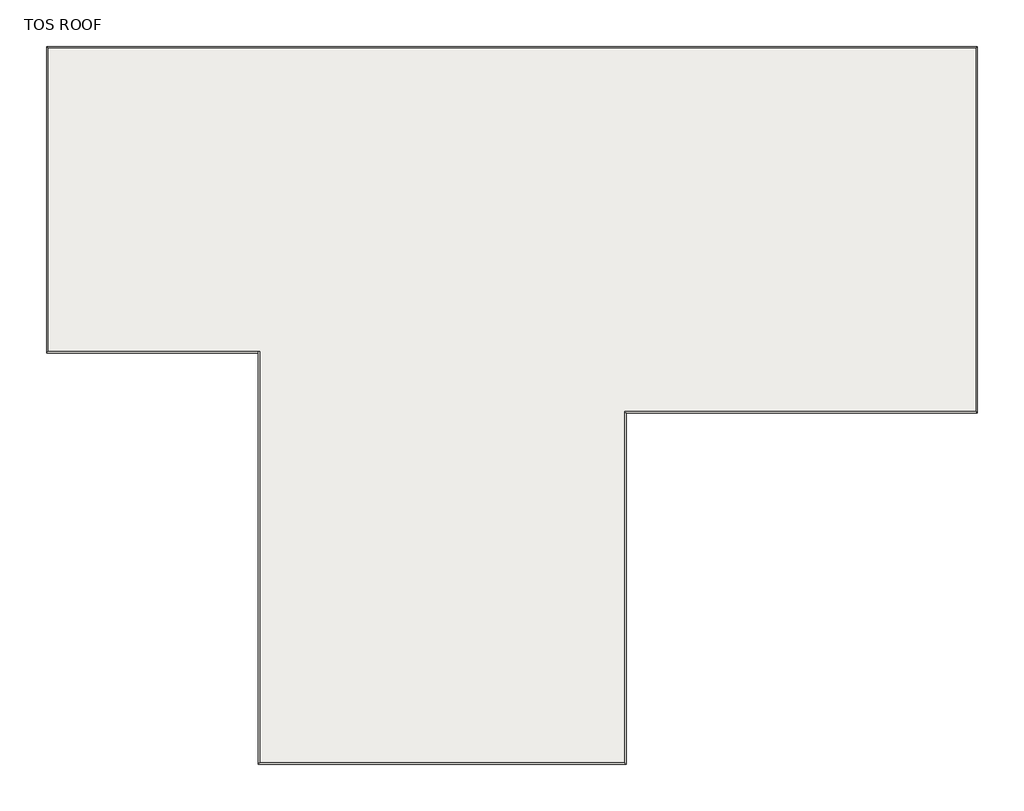
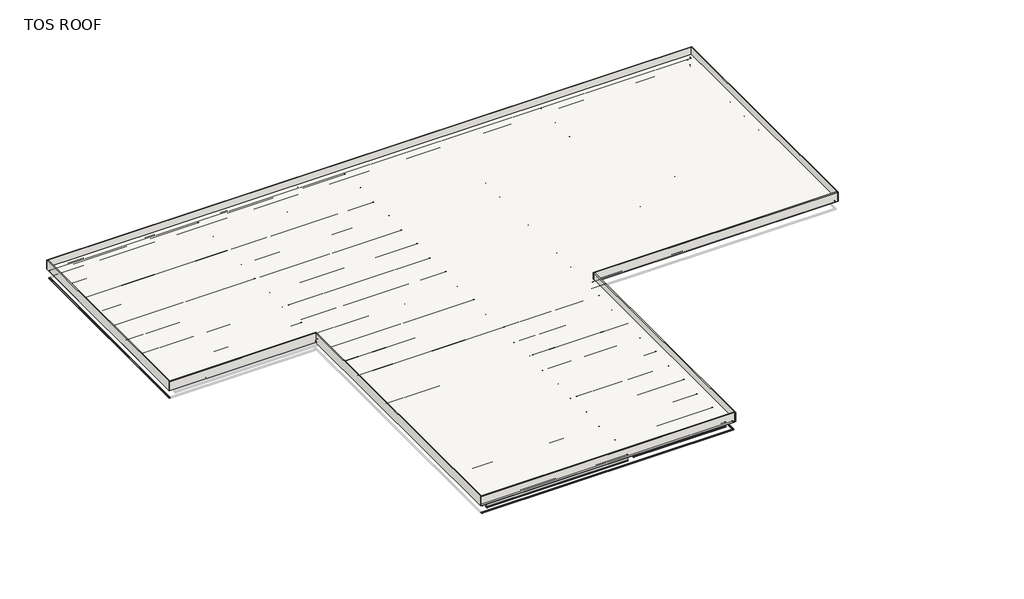
# One storey, part 1 of 3: 41 beams, 8 walls, 1 roof, 1 slab.
"""IFC4 building model written with IfcOpenShell, lengths in millimetres."""

import ifcopenshell
import ifcopenshell.guid

model = None  # the IFC model being written
_history = None  # IfcOwnerHistory: only IFC2X3 demands one
_inside = {}  # id of a spatial element -> (the spatial element, [elements in it])
_under = {}  # id of a project, library or spatial element -> (it, [spatial elements below it])
_declared = {}  # id of a project -> (the project, [libraries it declares])
_typed = {}  # id of a type object -> (the type object, [elements of that type])
_made_of = {}  # id of a material, layer set ... -> (it, [elements and type objects made of it])


def new_model(schema):
    """Start an empty IFC model of exactly this schema.

    Asked for "IFC4X3", IfcOpenShell would pick the latest addendum, in which some entities
    have other attributes; the version numbers below select the first issue.
    IFC2X3 requires an IfcOwnerHistory on every rooted entity: one is made here for all.
    """
    global model, _history
    if schema == "IFC4X3":
        model = ifcopenshell.file(schema_version=(4, 3, 0, 0))
    else:
        model = ifcopenshell.file(schema=schema)
    _inside.clear()
    _under.clear()
    _declared.clear()
    _typed.clear()
    _made_of.clear()
    _history = None
    if model.schema == "IFC2X3":
        org = make("IfcOrganization", Name="unknown")
        user = make(
            "IfcPersonAndOrganization",
            ThePerson=make("IfcPerson", FamilyName="unknown"),
            TheOrganization=org,
        )
        app = make(
            "IfcApplication",
            ApplicationDeveloper=org,
            Version="unknown",
            ApplicationFullName="unknown",
            ApplicationIdentifier="unknown",
        )
        _history = make(
            "IfcOwnerHistory",
            OwningUser=user,
            OwningApplication=app,
            ChangeAction="ADDED",
            CreationDate=0,
        )
    return model


def make(cls, **values):
    """One entity of the class cls with the attributes given. An attribute that is None is left unset."""
    return model.create_entity(
        cls, **{name: value for name, value in values.items() if value is not None}
    )


def rooted(cls, **values):
    """An entity with a GlobalId (a new one), such as an element, a storey or a relation."""
    return make(cls, GlobalId=ifcopenshell.guid.new(), OwnerHistory=_history, **values)


def si_unit(unit_type, name, prefix=None):
    """IfcSIUnit, for example si_unit("LENGTHUNIT", "METRE", prefix="MILLI")."""
    return make("IfcSIUnit", UnitType=unit_type, Prefix=prefix, Name=name)


def assignment(units):
    """IfcUnitAssignment: the units of a project."""
    return None if units is None else make("IfcUnitAssignment", Units=units)


def point(xyz):
    """IfcCartesianPoint."""
    return None if xyz is None else make("IfcCartesianPoint", Coordinates=xyz)


def direction(xyz):
    """IfcDirection."""
    return None if xyz is None else make("IfcDirection", DirectionRatios=xyz)


def frame(location, z_axis=None, x_axis=None):
    """IfcAxis2Placement3D, a coordinate frame: its origin and axes. An axis left out is left unset."""
    return make(
        "IfcAxis2Placement3D",
        Location=point(location),
        Axis=direction(z_axis),
        RefDirection=direction(x_axis),
    )


def frame_2d(location, x_axis=None):
    """IfcAxis2Placement2D, a coordinate frame in the plane: its origin and x axis."""
    return make(
        "IfcAxis2Placement2D", Location=point(location), RefDirection=direction(x_axis)
    )


def origin():
    """The frame at (0, 0, 0) with its axes left unset."""
    return frame((0.0, 0.0, 0.0))


def place(relative_to, where):
    """IfcLocalPlacement: puts the frame where relative to a parent placement (None: the world)."""
    return make(
        "IfcLocalPlacement", PlacementRelTo=relative_to, RelativePlacement=where
    )


def context(
    kind, dimensions, precision=None, world=None, true_north=None, identifier=None
):
    """IfcGeometricRepresentationContext, for example the 3D "Model" context."""
    return make(
        "IfcGeometricRepresentationContext",
        ContextIdentifier=identifier,
        ContextType=kind,
        CoordinateSpaceDimension=dimensions,
        Precision=precision,
        WorldCoordinateSystem=world,
        TrueNorth=true_north,
    )


def project(units=None, contexts=None):
    """IfcProject with its units and contexts."""
    return rooted(
        "IfcProject",
        Name="project",
        RepresentationContexts=contexts,
        UnitsInContext=assignment(units),
    )


def spatial(cls, under=None, at=None, **own):
    """A site, building, storey or space (cls), placed at a placement, below another one or the project."""
    s = rooted(cls, ObjectPlacement=at, **own)
    if under is not None:
        _under.setdefault(under.id(), (under, []))[1].append(s)
    return s


def polyline(points):
    """IfcPolyline through the points."""
    return make("IfcPolyline", Points=[point(p) for p in points])


def circle_curve(where, radius):
    """IfcCircle in the frame where."""
    return make("IfcCircle", Position=where, Radius=radius)


def trimmed(basis, trim1, trim2, sense, master):
    """IfcTrimmedCurve: the piece of a basis curve between two trims."""
    return make(
        "IfcTrimmedCurve",
        BasisCurve=basis,
        Trim1=trim1,
        Trim2=trim2,
        SenseAgreement=sense,
        MasterRepresentation=master,
    )


def segment(curve, same_sense, transition):
    """IfcCompositeCurveSegment."""
    return make(
        "IfcCompositeCurveSegment",
        Transition=transition,
        SameSense=same_sense,
        ParentCurve=curve,
    )


def composite_curve(segments, self_intersect=None):
    """IfcCompositeCurve: segments joined end to end."""
    return make("IfcCompositeCurve", Segments=segments, SelfIntersect=self_intersect)


def outline(outer, holes=None, kind="AREA"):
    """IfcArbitraryClosedProfileDef: a profile drawn as a closed curve; with holes, ...WithVoids."""
    if holes is None:
        return make("IfcArbitraryClosedProfileDef", ProfileType=kind, OuterCurve=outer)
    return make(
        "IfcArbitraryProfileDefWithVoids",
        ProfileType=kind,
        OuterCurve=outer,
        InnerCurves=holes,
    )


def extrude(swept, where, along, depth):
    """IfcExtrudedAreaSolid: the profile swept, set in the frame where, extruded along a direction by depth."""
    return make(
        "IfcExtrudedAreaSolid",
        SweptArea=swept,
        Position=where,
        ExtrudedDirection=direction(along),
        Depth=depth,
    )


def faces_of(points, faces, orient=None, outer=None):
    """IfcFace entities. A face is a list of loops; a loop is a list of indices into points, from 0.

    orient and outer hold one flag for each loop. By default every Orientation is true, the
    first loop of a face is its IfcFaceOuterBound and the others are IfcFaceBound.
    """
    made = []
    for i, loops in enumerate(faces):
        bounds = []
        for j, loop in enumerate(loops):
            is_outer = j == 0 if outer is None else outer[i][j]
            bounds.append(
                make(
                    "IfcFaceOuterBound" if is_outer else "IfcFaceBound",
                    Bound=make("IfcPolyLoop", Polygon=[points[k] for k in loop]),
                    Orientation=True if orient is None else orient[i][j],
                )
            )
        made.append(make("IfcFace", Bounds=bounds))
    return made


def faceted_brep(points, faces, orient=None, outer=None, voids=None):
    """IfcFacetedBrep: a solid bounded by flat faces; with voids (closed shells), ...WithVoids."""
    shared = [point(p) for p in points]
    hull = make("IfcClosedShell", CfsFaces=faces_of(shared, faces, orient, outer))
    if voids is None:
        return make("IfcFacetedBrep", Outer=hull)
    return make(
        "IfcFacetedBrepWithVoids",
        Outer=hull,
        Voids=[
            make(cls, CfsFaces=faces_of(shared, fs, o, b)) for cls, fs, o, b in voids
        ],
    )


def shape(context_of_items, identifier, shape_type, items):
    """IfcShapeRepresentation: the items that make up one representation, for example the "Body"."""
    return make(
        "IfcShapeRepresentation",
        ContextOfItems=context_of_items,
        RepresentationIdentifier=identifier,
        RepresentationType=shape_type,
        Items=items,
    )


def source(mapping_origin, context_of_items, identifier, shape_type, items):
    """IfcRepresentationMap: a shape defined once, which mapped items show again and again."""
    return make(
        "IfcRepresentationMap",
        MappingOrigin=mapping_origin,
        MappedRepresentation=shape(context_of_items, identifier, shape_type, items),
    )


def transform(
    local_origin,
    x_axis=None,
    y_axis=None,
    z_axis=None,
    scale=None,
    scale2=None,
    scale3=None,
    uniform=True,
):
    """IfcCartesianTransformationOperator3D, or its non-uniform kind. x_axis, y_axis, z_axis: its Axis1, 2, 3."""
    if uniform:
        return make(
            "IfcCartesianTransformationOperator3D",
            Axis1=direction(x_axis),
            Axis2=direction(y_axis),
            LocalOrigin=point(local_origin),
            Scale=scale,
            Axis3=direction(z_axis),
        )
    return make(
        "IfcCartesianTransformationOperator3DnonUniform",
        Axis1=direction(x_axis),
        Axis2=direction(y_axis),
        LocalOrigin=point(local_origin),
        Scale=scale,
        Axis3=direction(z_axis),
        Scale2=scale2,
        Scale3=scale3,
    )


def mapped(mapping_source, mapping_target):
    """IfcMappedItem: shows the shape of a source again, moved by a transform."""
    return make(
        "IfcMappedItem", MappingSource=mapping_source, MappingTarget=mapping_target
    )


def made_of(thing, what):
    """Note that an element or type object is made of a material, layer set ...; save() writes the relation."""
    if what is not None:
        _made_of.setdefault(what.id(), (what, []))[1].append(thing)
    return thing


def element(
    cls,
    number,
    at=None,
    inside=None,
    cuts=None,
    type_object=None,
    material=None,
    context=None,
    identifier="Body",
    shape_type=None,
    held_by="IfcProductDefinitionShape",
    body=None,
    shapes=None,
    **own,
):
    """One element of the class cls, such as IfcWall. Its Tag is "e" and its number.

    at: its placement. inside: the storey or other place that contains it. cuts: it is an
    opening in that element (IfcRelVoidsElement). A single representation is given by context,
    identifier, shape_type and body (its items); several are given by shapes. held_by: the class
    of the entity that holds the representations. save() writes the other relations.
    """
    e = rooted(cls, Tag="e%d" % number, ObjectPlacement=at, **own)
    if body is not None:
        shapes = [shape(context, identifier, shape_type, body)]
    if shapes is not None:
        e.Representation = make(held_by, Representations=shapes)
    if inside is not None:
        _inside.setdefault(inside.id(), (inside, []))[1].append(e)
    if cuts is not None:
        rooted(
            "IfcRelVoidsElement", RelatingBuildingElement=cuts, RelatedOpeningElement=e
        )
    if type_object is not None:
        _typed.setdefault(type_object.id(), (type_object, []))[1].append(e)
    return made_of(e, material)


def aggregate(whole, parts):
    """IfcRelAggregates: a whole, such as a stair, and the parts it consists of."""
    return rooted("IfcRelAggregates", RelatingObject=whole, RelatedObjects=parts)


def save(model, path):
    """Write the relations noted so far, then the file.

    IfcRelAggregates (storeys below a building ...), IfcRelContainedInSpatialStructure (elements
    in a storey), IfcRelDefinesByType, IfcRelAssociatesMaterial and IfcRelDeclares: one each for
    every whole, place, type object, material and project.
    """
    for whole, parts in _under.values():
        aggregate(whole, parts)
    for where, things in _inside.values():
        rooted(
            "IfcRelContainedInSpatialStructure",
            RelatedElements=things,
            RelatingStructure=where,
        )
    for kind, things in _typed.values():
        rooted("IfcRelDefinesByType", RelatedObjects=things, RelatingType=kind)
    for what, things in _made_of.values():
        rooted("IfcRelAssociatesMaterial", RelatedObjects=things, RelatingMaterial=what)
    for by, libraries in _declared.values():
        rooted("IfcRelDeclares", RelatingContext=by, RelatedDefinitions=libraries)
    model.write(path)


def beam_c270cd18(model_context):
    return source(origin(), model_context, "Body", "SweptSolid", [
        extrude(outline(composite_curve([segment(polyline([(75.0, -141.0), (75.0, -150.0), (-75.0, -150.0), (-75.0, -141.0), (-16.25, -141.0)]), True, "CONTINUOUS"), segment(trimmed(circle_curve(frame_2d((-16.25, -128.0)), 13.0), [point((-16.25, -141.0))], [point((-3.25, -128.0))], True, "CARTESIAN"), True, "CONTINUOUS"), segment(polyline([(-3.25, -128.0), (-3.25, 128.0)]), True, "CONTINUOUS"), segment(trimmed(circle_curve(frame_2d((-16.25, 128.0)), 13.0), [point((-3.25, 128.0))], [point((-16.25, 141.0))], True, "CARTESIAN"), True, "CONTINUOUS"), segment(polyline([(-16.25, 141.0), (-75.0, 141.0), (-75.0, 150.0), (75.0, 150.0), (75.0, 141.0), (16.25, 141.0)]), True, "CONTINUOUS"), segment(trimmed(circle_curve(frame_2d((16.25, 128.0)), 13.0), [point((16.25, 141.0))], [point((3.25, 128.0))], True, "CARTESIAN"), True, "CONTINUOUS"), segment(polyline([(3.25, 128.0), (3.25, -128.0)]), True, "CONTINUOUS"), segment(trimmed(circle_curve(frame_2d((16.25, -128.0)), 13.0), [point((3.25, -128.0))], [point((16.25, -141.0))], True, "CARTESIAN"), True, "CONTINUOUS"), segment(polyline([(16.25, -141.0), (75.0, -141.0)]), True, "CONTINUOUS")], self_intersect=False)), frame((-2837.3, 0.0, 0.0), z_axis=(1.0, 0.0, 0.0), x_axis=(0.0, 1.0, 0.0)), (0.0, 0.0, 1.0), 5674.6),
    ])


def beam_0d7a42ae(model_context):
    return source(origin(), model_context, "Body", "SweptSolid", [
        extrude(outline(composite_curve([segment(polyline([(100.0, -283.0), (100.0, -300.0), (-100.0, -300.0), (-100.0, -283.0), (-27.5, -283.0)]), True, "CONTINUOUS"), segment(trimmed(circle_curve(frame_2d((-27.5, -261.0)), 22.0), [point((-27.5, -283.0))], [point((-5.5, -261.0))], True, "CARTESIAN"), True, "CONTINUOUS"), segment(polyline([(-5.5, -261.0), (-5.5, 261.0)]), True, "CONTINUOUS"), segment(trimmed(circle_curve(frame_2d((-27.5, 261.0)), 22.0), [point((-5.5, 261.0))], [point((-27.5, 283.0))], True, "CARTESIAN"), True, "CONTINUOUS"), segment(polyline([(-27.5, 283.0), (-100.0, 283.0), (-100.0, 300.0), (100.0, 300.0), (100.0, 283.0), (27.5, 283.0)]), True, "CONTINUOUS"), segment(trimmed(circle_curve(frame_2d((27.5, 261.0)), 22.0), [point((27.5, 283.0))], [point((5.5, 261.0))], True, "CARTESIAN"), True, "CONTINUOUS"), segment(polyline([(5.5, 261.0), (5.5, -261.0)]), True, "CONTINUOUS"), segment(trimmed(circle_curve(frame_2d((27.5, -261.0)), 22.0), [point((5.5, -261.0))], [point((27.5, -283.0))], True, "CARTESIAN"), True, "CONTINUOUS"), segment(polyline([(27.5, -283.0), (100.0, -283.0)]), True, "CONTINUOUS")], self_intersect=False)), frame((-5912.3, 0.0, 0.0), z_axis=(1.0, 0.0, 0.0), x_axis=(0.0, 1.0, 0.0)), (0.0, 0.0, 1.0), 11749.6),
    ])


def beam_9fd407d8(model_context):
    return source(origin(), model_context, "Body", "SweptSolid", [
        extrude(outline(composite_curve([segment(polyline([(150.0, -374.0), (150.0, -400.0), (-150.0, -400.0), (-150.0, -374.0), (-35.0, -374.0)]), True, "CONTINUOUS"), segment(trimmed(circle_curve(frame_2d((-35.0, -346.0)), 28.0), [point((-35.0, -374.0))], [point((-7.0, -346.0))], True, "CARTESIAN"), True, "CONTINUOUS"), segment(polyline([(-7.0, -346.0), (-7.0, 346.0)]), True, "CONTINUOUS"), segment(trimmed(circle_curve(frame_2d((-35.0, 346.0)), 28.0), [point((-7.0, 346.0))], [point((-35.0, 374.0))], True, "CARTESIAN"), True, "CONTINUOUS"), segment(polyline([(-35.0, 374.0), (-150.0, 374.0), (-150.0, 400.0), (150.0, 400.0), (150.0, 374.0), (35.0, 374.0)]), True, "CONTINUOUS"), segment(trimmed(circle_curve(frame_2d((35.0, 346.0)), 28.0), [point((35.0, 374.0))], [point((7.0, 346.0))], True, "CARTESIAN"), True, "CONTINUOUS"), segment(polyline([(7.0, 346.0), (7.0, -346.0)]), True, "CONTINUOUS"), segment(trimmed(circle_curve(frame_2d((35.0, -346.0)), 28.0), [point((7.0, -346.0))], [point((35.0, -374.0))], True, "CARTESIAN"), True, "CONTINUOUS"), segment(polyline([(35.0, -374.0), (150.0, -374.0)]), True, "CONTINUOUS")], self_intersect=False)), frame((-8837.3, 0.0, 0.0), z_axis=(1.0, 0.0, 0.0), x_axis=(0.0, 1.0, 0.0)), (0.0, 0.0, 1.0), 17749.6),
    ])


def beam_a13b9fc3(model_context):
    return source(origin(), model_context, "Body", "SweptSolid", [
        extrude(outline(composite_curve([segment(polyline([(150.0, -374.0), (150.0, -400.0), (-150.0, -400.0), (-150.0, -374.0), (-35.0, -374.0)]), True, "CONTINUOUS"), segment(trimmed(circle_curve(frame_2d((-35.0, -346.0)), 28.0), [point((-35.0, -374.0))], [point((-7.0, -346.0))], True, "CARTESIAN"), True, "CONTINUOUS"), segment(polyline([(-7.0, -346.0), (-7.0, 346.0)]), True, "CONTINUOUS"), segment(trimmed(circle_curve(frame_2d((-35.0, 346.0)), 28.0), [point((-7.0, 346.0))], [point((-35.0, 374.0))], True, "CARTESIAN"), True, "CONTINUOUS"), segment(polyline([(-35.0, 374.0), (-150.0, 374.0), (-150.0, 400.0), (150.0, 400.0), (150.0, 374.0), (35.0, 374.0)]), True, "CONTINUOUS"), segment(trimmed(circle_curve(frame_2d((35.0, 346.0)), 28.0), [point((35.0, 374.0))], [point((7.0, 346.0))], True, "CARTESIAN"), True, "CONTINUOUS"), segment(polyline([(7.0, 346.0), (7.0, -346.0)]), True, "CONTINUOUS"), segment(trimmed(circle_curve(frame_2d((35.0, -346.0)), 28.0), [point((7.0, -346.0))], [point((35.0, -374.0))], True, "CARTESIAN"), True, "CONTINUOUS"), segment(polyline([(35.0, -374.0), (150.0, -374.0)]), True, "CONTINUOUS")], self_intersect=False)), frame((-8693.3, 0.0, 0.0), z_axis=(1.0, 0.0, 0.0), x_axis=(0.0, 1.0, 0.0)), (0.0, 0.0, 1.0), 17386.6),
    ])


def beam_fedc1a72(model_context):
    return source(origin(), model_context, "Body", "SweptSolid", [
        extrude(outline(composite_curve([segment(polyline([(100.0, -283.0), (100.0, -300.0), (-100.0, -300.0), (-100.0, -283.0), (-27.5, -283.0)]), True, "CONTINUOUS"), segment(trimmed(circle_curve(frame_2d((-27.5, -261.0)), 22.0), [point((-27.5, -283.0))], [point((-5.5, -261.0))], True, "CARTESIAN"), True, "CONTINUOUS"), segment(polyline([(-5.5, -261.0), (-5.5, 261.0)]), True, "CONTINUOUS"), segment(trimmed(circle_curve(frame_2d((-27.5, 261.0)), 22.0), [point((-5.5, 261.0))], [point((-27.5, 283.0))], True, "CARTESIAN"), True, "CONTINUOUS"), segment(polyline([(-27.5, 283.0), (-100.0, 283.0), (-100.0, 300.0), (100.0, 300.0), (100.0, 283.0), (27.5, 283.0)]), True, "CONTINUOUS"), segment(trimmed(circle_curve(frame_2d((27.5, 261.0)), 22.0), [point((27.5, 283.0))], [point((5.5, 261.0))], True, "CARTESIAN"), True, "CONTINUOUS"), segment(polyline([(5.5, 261.0), (5.5, -261.0)]), True, "CONTINUOUS"), segment(trimmed(circle_curve(frame_2d((27.5, -261.0)), 22.0), [point((5.5, -261.0))], [point((27.5, -283.0))], True, "CARTESIAN"), True, "CONTINUOUS"), segment(polyline([(27.5, -283.0), (100.0, -283.0)]), True, "CONTINUOUS")], self_intersect=False)), frame((-5693.3, 0.0, 0.0), z_axis=(1.0, 0.0, 0.0), x_axis=(0.0, 1.0, 0.0)), (0.0, 0.0, 1.0), 11386.6),
    ])


def steel_framing_lc_f9ca99c4(model_context):
    return source(origin(), model_context, "Body", "SweptSolid", [
        extrude(outline(composite_curve([segment(polyline([(18.6, 67.0), (18.6, -67.0)]), True, "CONTINUOUS"), segment(trimmed(circle_curve(frame_2d((10.6, -67.0)), 8.0), [point((18.6, -67.0))], [point((10.6, -75.0))], False, "CARTESIAN"), True, "CONTINUOUS"), segment(polyline([(10.6, -75.0), (-48.4, -75.0)]), True, "CONTINUOUS"), segment(trimmed(circle_curve(frame_2d((-48.4, -67.0)), 8.0), [point((-48.4, -75.0))], [point((-56.4, -67.0))], False, "CARTESIAN"), True, "CONTINUOUS"), segment(polyline([(-56.4, -67.0), (-56.4, -50.0), (-53.2, -50.0), (-53.2, -67.0)]), True, "CONTINUOUS"), segment(trimmed(circle_curve(frame_2d((-48.4, -67.0)), 4.8), [point((-53.2, -67.0))], [point((-48.4, -71.8))], True, "CARTESIAN"), True, "CONTINUOUS"), segment(polyline([(-48.4, -71.8), (10.6, -71.8)]), True, "CONTINUOUS"), segment(trimmed(circle_curve(frame_2d((10.6, -67.0)), 4.8), [point((10.6, -71.8))], [point((15.4, -67.0))], True, "CARTESIAN"), True, "CONTINUOUS"), segment(polyline([(15.4, -67.0), (15.4, 67.0)]), True, "CONTINUOUS"), segment(trimmed(circle_curve(frame_2d((10.6, 67.0)), 4.8), [point((15.4, 67.0))], [point((10.6, 71.8))], True, "CARTESIAN"), True, "CONTINUOUS"), segment(polyline([(10.6, 71.8), (-48.4, 71.8)]), True, "CONTINUOUS"), segment(trimmed(circle_curve(frame_2d((-48.4, 67.0)), 4.8), [point((-48.4, 71.8))], [point((-53.2, 67.0))], True, "CARTESIAN"), True, "CONTINUOUS"), segment(polyline([(-53.2, 67.0), (-53.2, 50.0), (-56.4, 50.0), (-56.4, 67.0)]), True, "CONTINUOUS"), segment(trimmed(circle_curve(frame_2d((-48.4, 67.0)), 8.0), [point((-56.4, 67.0))], [point((-48.4, 75.0))], False, "CARTESIAN"), True, "CONTINUOUS"), segment(polyline([(-48.4, 75.0), (10.6, 75.0)]), True, "CONTINUOUS"), segment(trimmed(circle_curve(frame_2d((10.6, 67.0)), 8.0), [point((10.6, 75.0))], [point((18.6, 67.0))], False, "CARTESIAN"), True, "CONTINUOUS")], self_intersect=False)), frame((-12797.0, 0.0, 0.0), z_axis=(1.0, 0.0, 0.0), x_axis=(0.0, 1.0, 0.0)), (0.0, 0.0, 1.0), 25581.0),
    ])


def steel_framing_lc_7a68255c(model_context):
    return source(origin(), model_context, "Body", "SweptSolid", [
        extrude(outline(composite_curve([segment(polyline([(18.6, 67.0), (18.6, -67.0)]), True, "CONTINUOUS"), segment(trimmed(circle_curve(frame_2d((10.6, -67.0)), 8.0), [point((18.6, -67.0))], [point((10.6, -75.0))], False, "CARTESIAN"), True, "CONTINUOUS"), segment(polyline([(10.6, -75.0), (-48.4, -75.0)]), True, "CONTINUOUS"), segment(trimmed(circle_curve(frame_2d((-48.4, -67.0)), 8.0), [point((-48.4, -75.0))], [point((-56.4, -67.0))], False, "CARTESIAN"), True, "CONTINUOUS"), segment(polyline([(-56.4, -67.0), (-56.4, -50.0), (-53.2, -50.0), (-53.2, -67.0)]), True, "CONTINUOUS"), segment(trimmed(circle_curve(frame_2d((-48.4, -67.0)), 4.8), [point((-53.2, -67.0))], [point((-48.4, -71.8))], True, "CARTESIAN"), True, "CONTINUOUS"), segment(polyline([(-48.4, -71.8), (10.6, -71.8)]), True, "CONTINUOUS"), segment(trimmed(circle_curve(frame_2d((10.6, -67.0)), 4.8), [point((10.6, -71.8))], [point((15.4, -67.0))], True, "CARTESIAN"), True, "CONTINUOUS"), segment(polyline([(15.4, -67.0), (15.4, 67.0)]), True, "CONTINUOUS"), segment(trimmed(circle_curve(frame_2d((10.6, 67.0)), 4.8), [point((15.4, 67.0))], [point((10.6, 71.8))], True, "CARTESIAN"), True, "CONTINUOUS"), segment(polyline([(10.6, 71.8), (-48.4, 71.8)]), True, "CONTINUOUS"), segment(trimmed(circle_curve(frame_2d((-48.4, 67.0)), 4.8), [point((-48.4, 71.8))], [point((-53.2, 67.0))], True, "CARTESIAN"), True, "CONTINUOUS"), segment(polyline([(-53.2, 67.0), (-53.2, 50.0), (-56.4, 50.0), (-56.4, 67.0)]), True, "CONTINUOUS"), segment(trimmed(circle_curve(frame_2d((-48.4, 67.0)), 8.0), [point((-56.4, 67.0))], [point((-48.4, 75.0))], False, "CARTESIAN"), True, "CONTINUOUS"), segment(polyline([(-48.4, 75.0), (10.6, 75.0)]), True, "CONTINUOUS"), segment(trimmed(circle_curve(frame_2d((10.6, 67.0)), 8.0), [point((10.6, 75.0))], [point((18.6, 67.0))], False, "CARTESIAN"), True, "CONTINUOUS")], self_intersect=False)), frame((-15450.0, 0.0, 0.0), z_axis=(1.0, 0.0, 0.0), x_axis=(0.0, 1.0, 0.0)), (0.0, 0.0, 1.0), 30900.0),
    ])


model = new_model("IFC4")

# Units and contexts
model_context = context("Model", 3, world=origin())
ifc_project = project(units=[si_unit("LENGTHUNIT", "METRE", prefix="MILLI")], contexts=[model_context])

# Site, building, storey
site = spatial("IfcSite", under=ifc_project)
building = spatial("IfcBuilding", under=site)
storey = spatial("IfcBuildingStorey", under=building, Name="TOS ROOF", Elevation=10199.9618634)

# Beams
placement = place(None, origin())
element("IfcBeam", 1, at=placement, inside=storey, context=model_context, shape_type="SweptSolid", body=[
    extrude(outline(composite_curve([segment(polyline([(9908.9618634, 36075.0), (9908.9618634, 36016.25)]), True, "CONTINUOUS"), segment(trimmed(circle_curve(frame_2d((9921.9618634, 36016.25)), 13.0), [point((9908.9618634, 36016.25))], [point((9921.9618634, 36003.25))], True, "CARTESIAN"), True, "CONTINUOUS"), segment(polyline([(9921.9618634, 36003.25), (10177.9618634, 36003.25)]), True, "CONTINUOUS"), segment(trimmed(circle_curve(frame_2d((10177.9618634, 36016.25)), 13.0), [point((10177.9618634, 36003.25))], [point((10190.9618634, 36016.25))], True, "CARTESIAN"), True, "CONTINUOUS"), segment(polyline([(10190.9618634, 36016.25), (10190.9618634, 36075.0), (10199.9618634, 36075.0), (10199.9618634, 35925.0), (10190.9618634, 35925.0), (10190.9618634, 35983.75)]), True, "CONTINUOUS"), segment(trimmed(circle_curve(frame_2d((10177.9618634, 35983.75)), 13.0), [point((10190.9618634, 35983.75))], [point((10177.9618634, 35996.75))], True, "CARTESIAN"), True, "CONTINUOUS"), segment(polyline([(10177.9618634, 35996.75), (9921.9618634, 35996.75)]), True, "CONTINUOUS"), segment(trimmed(circle_curve(frame_2d((9921.9618634, 35983.75)), 13.0), [point((9921.9618634, 35996.75))], [point((9908.9618634, 35983.75))], True, "CARTESIAN"), True, "CONTINUOUS"), segment(polyline([(9908.9618634, 35983.75), (9908.9618634, 35925.0), (9899.9618634, 35925.0), (9899.9618634, 36075.0), (9908.9618634, 36075.0)]), True, "CONTINUOUS")], self_intersect=False)), frame((0.0, -35837.3, 0.0), z_axis=(0.0, 1.0, 0.0), x_axis=(0.0, 0.0, 1.0)), (0.0, 0.0, 1.0), 5674.6),
])
element("IfcBeam", 2, at=placement, inside=storey, context=model_context, shape_type="SweptSolid", body=[
    extrude(outline(composite_curve([segment(polyline([(9908.9618634, 36075.0), (9908.9618634, 36016.25)]), True, "CONTINUOUS"), segment(trimmed(circle_curve(frame_2d((9921.9618634, 36016.25)), 13.0), [point((9908.9618634, 36016.25))], [point((9921.9618634, 36003.25))], True, "CARTESIAN"), True, "CONTINUOUS"), segment(polyline([(9921.9618634, 36003.25), (10177.9618634, 36003.25)]), True, "CONTINUOUS"), segment(trimmed(circle_curve(frame_2d((10177.9618634, 36016.25)), 13.0), [point((10177.9618634, 36003.25))], [point((10190.9618634, 36016.25))], True, "CARTESIAN"), True, "CONTINUOUS"), segment(polyline([(10190.9618634, 36016.25), (10190.9618634, 36075.0), (10199.9618634, 36075.0), (10199.9618634, 35925.0), (10190.9618634, 35925.0), (10190.9618634, 35983.75)]), True, "CONTINUOUS"), segment(trimmed(circle_curve(frame_2d((10177.9618634, 35983.75)), 13.0), [point((10190.9618634, 35983.75))], [point((10177.9618634, 35996.75))], True, "CARTESIAN"), True, "CONTINUOUS"), segment(polyline([(10177.9618634, 35996.75), (9921.9618634, 35996.75)]), True, "CONTINUOUS"), segment(trimmed(circle_curve(frame_2d((9921.9618634, 35983.75)), 13.0), [point((9921.9618634, 35996.75))], [point((9908.9618634, 35983.75))], True, "CARTESIAN"), True, "CONTINUOUS"), segment(polyline([(9908.9618634, 35983.75), (9908.9618634, 35925.0), (9899.9618634, 35925.0), (9899.9618634, 36075.0), (9908.9618634, 36075.0)]), True, "CONTINUOUS")], self_intersect=False)), frame((0.0, -41837.3, 0.0), z_axis=(0.0, 1.0, 0.0), x_axis=(0.0, 0.0, 1.0)), (0.0, 0.0, 1.0), 5674.6),
])
element("IfcBeam", 3, at=placement, inside=storey, context=model_context, shape_type="SweptSolid", body=[
    extrude(outline(composite_curve([segment(polyline([(9908.9618634, 36075.0), (9908.9618634, 36016.25)]), True, "CONTINUOUS"), segment(trimmed(circle_curve(frame_2d((9921.9618634, 36016.25)), 13.0), [point((9908.9618634, 36016.25))], [point((9921.9618634, 36003.25))], True, "CARTESIAN"), True, "CONTINUOUS"), segment(polyline([(9921.9618634, 36003.25), (10177.9618634, 36003.25)]), True, "CONTINUOUS"), segment(trimmed(circle_curve(frame_2d((10177.9618634, 36016.25)), 13.0), [point((10177.9618634, 36003.25))], [point((10190.9618634, 36016.25))], True, "CARTESIAN"), True, "CONTINUOUS"), segment(polyline([(10190.9618634, 36016.25), (10190.9618634, 36075.0), (10199.9618634, 36075.0), (10199.9618634, 35925.0), (10190.9618634, 35925.0), (10190.9618634, 35983.75)]), True, "CONTINUOUS"), segment(trimmed(circle_curve(frame_2d((10177.9618634, 35983.75)), 13.0), [point((10190.9618634, 35983.75))], [point((10177.9618634, 35996.75))], True, "CARTESIAN"), True, "CONTINUOUS"), segment(polyline([(10177.9618634, 35996.75), (9921.9618634, 35996.75)]), True, "CONTINUOUS"), segment(trimmed(circle_curve(frame_2d((9921.9618634, 35983.75)), 13.0), [point((9921.9618634, 35996.75))], [point((9908.9618634, 35983.75))], True, "CARTESIAN"), True, "CONTINUOUS"), segment(polyline([(9908.9618634, 35983.75), (9908.9618634, 35925.0), (9899.9618634, 35925.0), (9899.9618634, 36075.0), (9908.9618634, 36075.0)]), True, "CONTINUOUS")], self_intersect=False)), frame((0.0, -47837.3, 0.0), z_axis=(0.0, 1.0, 0.0), x_axis=(0.0, 0.0, 1.0)), (0.0, 0.0, 1.0), 5674.6),
])
element("IfcBeam", 4, at=placement, inside=storey, context=model_context, shape_type="SweptSolid", body=[
    extrude(outline(composite_curve([segment(polyline([(-32850.0, 9425.9618634), (-32850.0, 9399.9618634), (-33150.0, 9399.9618634), (-33150.0, 9425.9618634), (-33035.0, 9425.9618634)]), True, "CONTINUOUS"), segment(trimmed(circle_curve(frame_2d((-33035.0, 9453.9618634)), 28.0), [point((-33035.0, 9425.9618634))], [point((-33007.0, 9453.9618634))], True, "CARTESIAN"), True, "CONTINUOUS"), segment(polyline([(-33007.0, 9453.9618634), (-33007.0, 10145.9618634)]), True, "CONTINUOUS"), segment(trimmed(circle_curve(frame_2d((-33035.0, 10145.9618634)), 28.0), [point((-33007.0, 10145.9618634))], [point((-33035.0, 10173.9618634))], True, "CARTESIAN"), True, "CONTINUOUS"), segment(polyline([(-33035.0, 10173.9618634), (-33150.0, 10173.9618634), (-33150.0, 10199.9618634), (-32850.0, 10199.9618634), (-32850.0, 10173.9618634), (-32965.0, 10173.9618634)]), True, "CONTINUOUS"), segment(trimmed(circle_curve(frame_2d((-32965.0, 10145.9618634)), 28.0), [point((-32965.0, 10173.9618634))], [point((-32993.0, 10145.9618634))], True, "CARTESIAN"), True, "CONTINUOUS"), segment(polyline([(-32993.0, 10145.9618634), (-32993.0, 9453.9618634)]), True, "CONTINUOUS"), segment(trimmed(circle_curve(frame_2d((-32965.0, 9453.9618634)), 28.0), [point((-32993.0, 9453.9618634))], [point((-32965.0, 9425.9618634))], True, "CARTESIAN"), True, "CONTINUOUS"), segment(polyline([(-32965.0, 9425.9618634), (-32850.0, 9425.9618634)]), True, "CONTINUOUS")], self_intersect=False)), frame((18162.7, 0.0, 0.0), z_axis=(1.0, 0.0, 0.0), x_axis=(0.0, 1.0, 0.0)), (0.0, 0.0, 1.0), 17749.6),
])
element("IfcBeam", 5, at=placement, inside=storey, context=model_context, shape_type="SweptSolid", body=[
    extrude(outline(composite_curve([segment(polyline([(-38850.0, 9425.9618634), (-38850.0, 9399.9618634), (-39150.0, 9399.9618634), (-39150.0, 9425.9618634), (-39035.0, 9425.9618634)]), True, "CONTINUOUS"), segment(trimmed(circle_curve(frame_2d((-39035.0, 9453.9618634)), 28.0), [point((-39035.0, 9425.9618634))], [point((-39007.0, 9453.9618634))], True, "CARTESIAN"), True, "CONTINUOUS"), segment(polyline([(-39007.0, 9453.9618634), (-39007.0, 10145.9618634)]), True, "CONTINUOUS"), segment(trimmed(circle_curve(frame_2d((-39035.0, 10145.9618634)), 28.0), [point((-39007.0, 10145.9618634))], [point((-39035.0, 10173.9618634))], True, "CARTESIAN"), True, "CONTINUOUS"), segment(polyline([(-39035.0, 10173.9618634), (-39150.0, 10173.9618634), (-39150.0, 10199.9618634), (-38850.0, 10199.9618634), (-38850.0, 10173.9618634), (-38965.0, 10173.9618634)]), True, "CONTINUOUS"), segment(trimmed(circle_curve(frame_2d((-38965.0, 10145.9618634)), 28.0), [point((-38965.0, 10173.9618634))], [point((-38993.0, 10145.9618634))], True, "CARTESIAN"), True, "CONTINUOUS"), segment(polyline([(-38993.0, 10145.9618634), (-38993.0, 9453.9618634)]), True, "CONTINUOUS"), segment(trimmed(circle_curve(frame_2d((-38965.0, 9453.9618634)), 28.0), [point((-38993.0, 9453.9618634))], [point((-38965.0, 9425.9618634))], True, "CARTESIAN"), True, "CONTINUOUS"), segment(polyline([(-38965.0, 9425.9618634), (-38850.0, 9425.9618634)]), True, "CONTINUOUS")], self_intersect=False)), frame((18162.7, 0.0, 0.0), z_axis=(1.0, 0.0, 0.0), x_axis=(0.0, 1.0, 0.0)), (0.0, 0.0, 1.0), 17749.6),
])
element("IfcBeam", 6, at=placement, inside=storey, context=model_context, shape_type="SweptSolid", body=[
    extrude(outline(composite_curve([segment(polyline([(-44850.0, 9425.9618634), (-44850.0, 9399.9618634), (-45150.0, 9399.9618634), (-45150.0, 9425.9618634), (-45035.0, 9425.9618634)]), True, "CONTINUOUS"), segment(trimmed(circle_curve(frame_2d((-45035.0, 9453.9618634)), 28.0), [point((-45035.0, 9425.9618634))], [point((-45007.0, 9453.9618634))], True, "CARTESIAN"), True, "CONTINUOUS"), segment(polyline([(-45007.0, 9453.9618634), (-45007.0, 10145.9618634)]), True, "CONTINUOUS"), segment(trimmed(circle_curve(frame_2d((-45035.0, 10145.9618634)), 28.0), [point((-45007.0, 10145.9618634))], [point((-45035.0, 10173.9618634))], True, "CARTESIAN"), True, "CONTINUOUS"), segment(polyline([(-45035.0, 10173.9618634), (-45150.0, 10173.9618634), (-45150.0, 10199.9618634), (-44850.0, 10199.9618634), (-44850.0, 10173.9618634), (-44965.0, 10173.9618634)]), True, "CONTINUOUS"), segment(trimmed(circle_curve(frame_2d((-44965.0, 10145.9618634)), 28.0), [point((-44965.0, 10173.9618634))], [point((-44993.0, 10145.9618634))], True, "CARTESIAN"), True, "CONTINUOUS"), segment(polyline([(-44993.0, 10145.9618634), (-44993.0, 9453.9618634)]), True, "CONTINUOUS"), segment(trimmed(circle_curve(frame_2d((-44965.0, 9453.9618634)), 28.0), [point((-44993.0, 9453.9618634))], [point((-44965.0, 9425.9618634))], True, "CARTESIAN"), True, "CONTINUOUS"), segment(polyline([(-44965.0, 9425.9618634), (-44850.0, 9425.9618634)]), True, "CONTINUOUS")], self_intersect=False)), frame((18162.7, 0.0, 0.0), z_axis=(1.0, 0.0, 0.0), x_axis=(0.0, 1.0, 0.0)), (0.0, 0.0, 1.0), 17749.6),
])
element("IfcBeam", 7, at=placement, inside=storey, context=model_context, shape_type="SweptSolid", body=[
    extrude(outline(composite_curve([segment(polyline([(9908.9618634, 48075.0), (9908.9618634, 48016.25)]), True, "CONTINUOUS"), segment(trimmed(circle_curve(frame_2d((9921.9618634, 48016.25)), 13.0), [point((9908.9618634, 48016.25))], [point((9921.9618634, 48003.25))], True, "CARTESIAN"), True, "CONTINUOUS"), segment(polyline([(9921.9618634, 48003.25), (10177.9618634, 48003.25)]), True, "CONTINUOUS"), segment(trimmed(circle_curve(frame_2d((10177.9618634, 48016.25)), 13.0), [point((10177.9618634, 48003.25))], [point((10190.9618634, 48016.25))], True, "CARTESIAN"), True, "CONTINUOUS"), segment(polyline([(10190.9618634, 48016.25), (10190.9618634, 48075.0), (10199.9618634, 48075.0), (10199.9618634, 47925.0), (10190.9618634, 47925.0), (10190.9618634, 47983.75)]), True, "CONTINUOUS"), segment(trimmed(circle_curve(frame_2d((10177.9618634, 47983.75)), 13.0), [point((10190.9618634, 47983.75))], [point((10177.9618634, 47996.75))], True, "CARTESIAN"), True, "CONTINUOUS"), segment(polyline([(10177.9618634, 47996.75), (9921.9618634, 47996.75)]), True, "CONTINUOUS"), segment(trimmed(circle_curve(frame_2d((9921.9618634, 47983.75)), 13.0), [point((9921.9618634, 47996.75))], [point((9908.9618634, 47983.75))], True, "CARTESIAN"), True, "CONTINUOUS"), segment(polyline([(9908.9618634, 47983.75), (9908.9618634, 47925.0), (9899.9618634, 47925.0), (9899.9618634, 48075.0), (9908.9618634, 48075.0)]), True, "CONTINUOUS")], self_intersect=False)), frame((0.0, -35837.3, 0.0), z_axis=(0.0, 1.0, 0.0), x_axis=(0.0, 0.0, 1.0)), (0.0, 0.0, 1.0), 5530.6),
])
element("IfcBeam", 8, at=placement, inside=storey, context=model_context, shape_type="SweptSolid", body=[
    extrude(outline(composite_curve([segment(polyline([(9908.9618634, 48075.0), (9908.9618634, 48016.25)]), True, "CONTINUOUS"), segment(trimmed(circle_curve(frame_2d((9921.9618634, 48016.25)), 13.0), [point((9908.9618634, 48016.25))], [point((9921.9618634, 48003.25))], True, "CARTESIAN"), True, "CONTINUOUS"), segment(polyline([(9921.9618634, 48003.25), (10177.9618634, 48003.25)]), True, "CONTINUOUS"), segment(trimmed(circle_curve(frame_2d((10177.9618634, 48016.25)), 13.0), [point((10177.9618634, 48003.25))], [point((10190.9618634, 48016.25))], True, "CARTESIAN"), True, "CONTINUOUS"), segment(polyline([(10190.9618634, 48016.25), (10190.9618634, 48075.0), (10199.9618634, 48075.0), (10199.9618634, 47925.0), (10190.9618634, 47925.0), (10190.9618634, 47983.75)]), True, "CONTINUOUS"), segment(trimmed(circle_curve(frame_2d((10177.9618634, 47983.75)), 13.0), [point((10190.9618634, 47983.75))], [point((10177.9618634, 47996.75))], True, "CARTESIAN"), True, "CONTINUOUS"), segment(polyline([(10177.9618634, 47996.75), (9921.9618634, 47996.75)]), True, "CONTINUOUS"), segment(trimmed(circle_curve(frame_2d((9921.9618634, 47983.75)), 13.0), [point((9921.9618634, 47996.75))], [point((9908.9618634, 47983.75))], True, "CARTESIAN"), True, "CONTINUOUS"), segment(polyline([(9908.9618634, 47983.75), (9908.9618634, 47925.0), (9899.9618634, 47925.0), (9899.9618634, 48075.0), (9908.9618634, 48075.0)]), True, "CONTINUOUS")], self_intersect=False)), frame((0.0, -47837.3, 0.0), z_axis=(0.0, 1.0, 0.0), x_axis=(0.0, 0.0, 1.0)), (0.0, 0.0, 1.0), 5674.6),
])
element("IfcBeam", 9, at=placement, inside=storey, context=model_context, shape_type="SweptSolid", body=[
    extrude(outline(composite_curve([segment(polyline([(-44900.0, 9616.9618634), (-44900.0, 9599.9618634), (-45100.0, 9599.9618634), (-45100.0, 9616.9618634), (-45027.5, 9616.9618634)]), True, "CONTINUOUS"), segment(trimmed(circle_curve(frame_2d((-45027.5, 9638.9618634)), 22.0), [point((-45027.5, 9616.9618634))], [point((-45005.5, 9638.9618634))], True, "CARTESIAN"), True, "CONTINUOUS"), segment(polyline([(-45005.5, 9638.9618634), (-45005.5, 10160.9618634)]), True, "CONTINUOUS"), segment(trimmed(circle_curve(frame_2d((-45027.5, 10160.9618634)), 22.0), [point((-45005.5, 10160.9618634))], [point((-45027.5, 10182.9618634))], True, "CARTESIAN"), True, "CONTINUOUS"), segment(polyline([(-45027.5, 10182.9618634), (-45100.0, 10182.9618634), (-45100.0, 10199.9618634), (-44900.0, 10199.9618634), (-44900.0, 10182.9618634), (-44972.5, 10182.9618634)]), True, "CONTINUOUS"), segment(trimmed(circle_curve(frame_2d((-44972.5, 10160.9618634)), 22.0), [point((-44972.5, 10182.9618634))], [point((-44994.5, 10160.9618634))], True, "CARTESIAN"), True, "CONTINUOUS"), segment(polyline([(-44994.5, 10160.9618634), (-44994.5, 9638.9618634)]), True, "CONTINUOUS"), segment(trimmed(circle_curve(frame_2d((-44972.5, 9638.9618634)), 22.0), [point((-44994.5, 9638.9618634))], [point((-44972.5, 9616.9618634))], True, "CARTESIAN"), True, "CONTINUOUS"), segment(polyline([(-44972.5, 9616.9618634), (-44900.0, 9616.9618634)]), True, "CONTINUOUS")], self_intersect=False)), frame((36087.7, 0.0, 0.0), z_axis=(1.0, 0.0, 0.0), x_axis=(0.0, 1.0, 0.0)), (0.0, 0.0, 1.0), 11749.6),
])
beam_shape = beam_c270cd18(model_context)
element("IfcBeam", 10, at=placement, inside=storey, context=model_context, shape_type="MappedRepresentation", body=[
    mapped(beam_shape, transform((18000.0, -33000.0, 10049.9618634), x_axis=(0.0, -1.0, 0.0), y_axis=(1.0, 0.0, 0.0), z_axis=(0.0, 0.0, 1.0))),
])
element("IfcBeam", 11, at=placement, inside=storey, context=model_context, shape_type="MappedRepresentation", body=[
    mapped(beam_shape, transform((18000.0, -39000.0, 10049.9618634), x_axis=(0.0, -1.0, 0.0), y_axis=(1.0, 0.0, 0.0), z_axis=(0.0, 0.0, 1.0))),
])
element("IfcBeam", 12, at=placement, inside=storey, context=model_context, shape_type="MappedRepresentation", body=[
    mapped(beam_shape, transform((18000.0, -45000.0, 10049.9618634), x_axis=(0.0, -1.0, 0.0), y_axis=(1.0, 0.0, 0.0), z_axis=(0.0, 0.0, 1.0))),
])
element("IfcBeam", 13, at=placement, inside=storey, context=model_context, shape_type="MappedRepresentation", body=[
    mapped(beam_shape, transform((18000.0, -51000.0, 10049.9618634), x_axis=(0.0, -1.0, 0.0), y_axis=(1.0, 0.0, 0.0), z_axis=(0.0, 0.0, 1.0))),
])
element("IfcBeam", 14, at=placement, inside=storey, context=model_context, shape_type="MappedRepresentation", body=[
    mapped(beam_shape, transform((18000.0, -57000.0, 10049.9618634), x_axis=(0.0, -1.0, 0.0), y_axis=(1.0, 0.0, 0.0), z_axis=(0.0, 0.0, 1.0))),
])
element("IfcBeam", 15, at=placement, inside=storey, context=model_context, shape_type="MappedRepresentation", body=[
    mapped(beam_shape, transform((36000.0, -51000.0, 10049.9618634), x_axis=(0.0, -1.0, 0.0), y_axis=(1.0, 0.0, 0.0), z_axis=(0.0, 0.0, 1.0))),
])
element("IfcBeam", 16, at=placement, inside=storey, context=model_context, shape_type="MappedRepresentation", body=[
    mapped(beam_shape, transform((36000.0, -57000.0, 10049.9618634), x_axis=(0.0, -1.0, 0.0), y_axis=(1.0, 0.0, 0.0), z_axis=(0.0, 0.0, 1.0))),
])
element("IfcBeam", 17, at=placement, inside=storey, context=model_context, shape_type="MappedRepresentation", body=[
    mapped(beam_shape, transform((48000.0, -39000.0, 10049.9618634), x_axis=(0.0, -1.0, 0.0), y_axis=(1.0, 0.0, 0.0), z_axis=(0.0, 0.0, 1.0))),
])
element("IfcBeam", 18, at=placement, inside=storey, context=model_context, shape_type="MappedRepresentation", body=[
    mapped(beam_shape, transform((48000.0, -51000.0, 10049.9618634), x_axis=(0.0, -1.0, 0.0), y_axis=(1.0, 0.0, 0.0), z_axis=(0.0, 0.0, 1.0))),
])
element("IfcBeam", 19, at=placement, inside=storey, context=model_context, shape_type="MappedRepresentation", body=[
    mapped(beam_shape, transform((48000.0, -57000.0, 10049.9618634), x_axis=(0.0, -1.0, 0.0), y_axis=(1.0, 0.0, 0.0), z_axis=(0.0, 0.0, 1.0))),
])
beam_2_shape = beam_0d7a42ae(model_context)
element("IfcBeam", 20, at=placement, inside=storey, context=model_context, shape_type="MappedRepresentation", body=[
    mapped(beam_2_shape, transform((42000.0, -57000.0, 9899.9618634), x_axis=(1.0, 0.0, 0.0), y_axis=(0.0, 1.0, 0.0), z_axis=(0.0, 0.0, 1.0))),
])
element("IfcBeam", 21, at=placement, inside=storey, context=model_context, shape_type="MappedRepresentation", body=[
    mapped(beam_2_shape, transform((42000.0, -51000.0, 9899.9618634), x_axis=(1.0, 0.0, 0.0), y_axis=(0.0, 1.0, 0.0), z_axis=(0.0, 0.0, 1.0))),
])
element("IfcBeam", 22, at=placement, inside=storey, context=model_context, shape_type="MappedRepresentation", body=[
    mapped(beam_2_shape, transform((42000.0, -39000.0, 9899.9618634), x_axis=(1.0, 0.0, 0.0), y_axis=(0.0, 1.0, 0.0), z_axis=(0.0, 0.0, 1.0))),
])
element("IfcBeam", 23, at=placement, inside=storey, context=model_context, shape_type="MappedRepresentation", body=[
    mapped(beam_2_shape, transform((42000.0, -33000.0, 9899.9618634), x_axis=(1.0, 0.0, 0.0), y_axis=(0.0, 1.0, 0.0), z_axis=(0.0, 0.0, 1.0))),
])
beam_3_shape = beam_9fd407d8(model_context)
element("IfcBeam", 24, at=placement, inside=storey, context=model_context, shape_type="MappedRepresentation", body=[
    mapped(beam_3_shape, transform((27000.0, -51000.0, 9799.9618634), x_axis=(1.0, 0.0, 0.0), y_axis=(0.0, 1.0, 0.0), z_axis=(0.0, 0.0, 1.0))),
])
element("IfcBeam", 25, at=placement, inside=storey, context=model_context, shape_type="MappedRepresentation", body=[
    mapped(beam_3_shape, transform((27000.0, -57000.0, 9799.9618634), x_axis=(1.0, 0.0, 0.0), y_axis=(0.0, 1.0, 0.0), z_axis=(0.0, 0.0, 1.0))),
])
beam_4_shape = beam_a13b9fc3(model_context)
element("IfcBeam", 26, at=placement, inside=storey, context=model_context, shape_type="MappedRepresentation", body=[
    mapped(beam_4_shape, transform((27000.0, -36000.0, 9799.9618634), x_axis=(1.0, 0.0, 0.0), y_axis=(0.0, 1.0, 0.0), z_axis=(0.0, 0.0, 1.0))),
])
element("IfcBeam", 27, at=placement, inside=storey, context=model_context, shape_type="MappedRepresentation", body=[
    mapped(beam_4_shape, transform((27000.0, -42000.0, 9799.9618634), x_axis=(1.0, 0.0, 0.0), y_axis=(0.0, 1.0, 0.0), z_axis=(0.0, 0.0, 1.0))),
])
element("IfcBeam", 28, at=placement, inside=storey, context=model_context, shape_type="MappedRepresentation", body=[
    mapped(beam_4_shape, transform((27000.0, -48000.0, 9799.9618634), x_axis=(1.0, 0.0, 0.0), y_axis=(0.0, 1.0, 0.0), z_axis=(0.0, 0.0, 1.0))),
])
element("IfcBeam", 29, at=placement, inside=storey, context=model_context, shape_type="MappedRepresentation", body=[
    mapped(beam_4_shape, transform((27000.0, -54000.0, 9799.9618634), x_axis=(1.0, 0.0, 0.0), y_axis=(0.0, 1.0, 0.0), z_axis=(0.0, 0.0, 1.0))),
])
element("IfcBeam", 30, at=placement, inside=storey, context=model_context, shape_type="MappedRepresentation", body=[
    mapped(beam_4_shape, transform((27000.0, -60000.0, 9799.9618634), x_axis=(1.0, 0.0, 0.0), y_axis=(0.0, 1.0, 0.0), z_axis=(0.0, 0.0, 1.0))),
])
beam_5_shape = beam_fedc1a72(model_context)
element("IfcBeam", 31, at=placement, inside=storey, context=model_context, shape_type="MappedRepresentation", body=[
    mapped(beam_5_shape, transform((42000.0, -60000.0, 9899.9618634), x_axis=(1.0, 0.0, 0.0), y_axis=(0.0, 1.0, 0.0), z_axis=(0.0, 0.0, 1.0))),
])
element("IfcBeam", 32, at=placement, inside=storey, context=model_context, shape_type="MappedRepresentation", body=[
    mapped(beam_5_shape, transform((42000.0, -54000.0, 9899.9618634), x_axis=(1.0, 0.0, 0.0), y_axis=(0.0, 1.0, 0.0), z_axis=(0.0, 0.0, 1.0))),
])
element("IfcBeam", 33, at=placement, inside=storey, context=model_context, shape_type="MappedRepresentation", body=[
    mapped(beam_5_shape, transform((42000.0, -48000.0, 9899.9618634), x_axis=(1.0, 0.0, 0.0), y_axis=(0.0, 1.0, 0.0), z_axis=(0.0, 0.0, 1.0))),
])
element("IfcBeam", 34, at=placement, inside=storey, context=model_context, shape_type="MappedRepresentation", body=[
    mapped(beam_5_shape, transform((42000.0, -42000.0, 9899.9618634), x_axis=(1.0, 0.0, 0.0), y_axis=(0.0, 1.0, 0.0), z_axis=(0.0, 0.0, 1.0))),
])
element("IfcBeam", 35, at=placement, inside=storey, context=model_context, shape_type="MappedRepresentation", body=[
    mapped(beam_5_shape, transform((42000.0, -36000.0, 9899.9618634), x_axis=(1.0, 0.0, 0.0), y_axis=(0.0, 1.0, 0.0), z_axis=(0.0, 0.0, 1.0))),
])
element("IfcBeam", 36, ObjectType="Steel Framing_LC", at=placement, inside=storey, context=model_context, shape_type="SweptSolid", body=[
    extrude(outline(composite_curve([segment(polyline([(9168.5618634, 48517.0), (9168.5618634, 48383.0)]), True, "CONTINUOUS"), segment(trimmed(circle_curve(frame_2d((9160.5618634, 48383.0)), 8.0), [point((9168.5618634, 48383.0))], [point((9160.5618634, 48375.0))], False, "CARTESIAN"), True, "CONTINUOUS"), segment(polyline([(9160.5618634, 48375.0), (9101.5618634, 48375.0)]), True, "CONTINUOUS"), segment(trimmed(circle_curve(frame_2d((9101.5618634, 48383.0)), 8.0), [point((9101.5618634, 48375.0))], [point((9093.5618634, 48383.0))], False, "CARTESIAN"), True, "CONTINUOUS"), segment(polyline([(9093.5618634, 48383.0), (9093.5618634, 48400.0), (9096.7618634, 48400.0), (9096.7618634, 48383.0)]), True, "CONTINUOUS"), segment(trimmed(circle_curve(frame_2d((9101.5618634, 48383.0)), 4.8), [point((9096.7618634, 48383.0))], [point((9101.5618634, 48378.2))], True, "CARTESIAN"), True, "CONTINUOUS"), segment(polyline([(9101.5618634, 48378.2), (9160.5618634, 48378.2)]), True, "CONTINUOUS"), segment(trimmed(circle_curve(frame_2d((9160.5618634, 48383.0)), 4.8), [point((9160.5618634, 48378.2))], [point((9165.3618634, 48383.0))], True, "CARTESIAN"), True, "CONTINUOUS"), segment(polyline([(9165.3618634, 48383.0), (9165.3618634, 48517.0)]), True, "CONTINUOUS"), segment(trimmed(circle_curve(frame_2d((9160.5618634, 48517.0)), 4.8), [point((9165.3618634, 48517.0))], [point((9160.5618634, 48521.8))], True, "CARTESIAN"), True, "CONTINUOUS"), segment(polyline([(9160.5618634, 48521.8), (9101.5618634, 48521.8)]), True, "CONTINUOUS"), segment(trimmed(circle_curve(frame_2d((9101.5618634, 48517.0)), 4.8), [point((9101.5618634, 48521.8))], [point((9096.7618634, 48517.0))], True, "CARTESIAN"), True, "CONTINUOUS"), segment(polyline([(9096.7618634, 48517.0), (9096.7618634, 48500.0), (9093.5618634, 48500.0), (9093.5618634, 48517.0)]), True, "CONTINUOUS"), segment(trimmed(circle_curve(frame_2d((9101.5618634, 48517.0)), 8.0), [point((9093.5618634, 48517.0))], [point((9101.5618634, 48525.0))], False, "CARTESIAN"), True, "CONTINUOUS"), segment(polyline([(9101.5618634, 48525.0), (9160.5618634, 48525.0)]), True, "CONTINUOUS"), segment(trimmed(circle_curve(frame_2d((9160.5618634, 48517.0)), 8.0), [point((9160.5618634, 48525.0))], [point((9168.5618634, 48517.0))], False, "CARTESIAN"), True, "CONTINUOUS")], self_intersect=False)), frame((0.0, -60300.0, 0.0), z_axis=(0.0, 1.0, 0.0), x_axis=(0.0, 0.0, 1.0)), (0.0, 0.0, 1.0), 29975.0),
])
element("IfcBeam", 37, ObjectType="Steel Framing_LC", at=placement, inside=storey, context=model_context, shape_type="SweptSolid", body=[
    extrude(outline(composite_curve([segment(polyline([(10168.5618634, 48517.0), (10168.5618634, 48383.0)]), True, "CONTINUOUS"), segment(trimmed(circle_curve(frame_2d((10160.5618634, 48383.0)), 8.0), [point((10168.5618634, 48383.0))], [point((10160.5618634, 48375.0))], False, "CARTESIAN"), True, "CONTINUOUS"), segment(polyline([(10160.5618634, 48375.0), (10101.5618634, 48375.0)]), True, "CONTINUOUS"), segment(trimmed(circle_curve(frame_2d((10101.5618634, 48383.0)), 8.0), [point((10101.5618634, 48375.0))], [point((10093.5618634, 48383.0))], False, "CARTESIAN"), True, "CONTINUOUS"), segment(polyline([(10093.5618634, 48383.0), (10093.5618634, 48400.0), (10096.7618634, 48400.0), (10096.7618634, 48383.0)]), True, "CONTINUOUS"), segment(trimmed(circle_curve(frame_2d((10101.5618634, 48383.0)), 4.8), [point((10096.7618634, 48383.0))], [point((10101.5618634, 48378.2))], True, "CARTESIAN"), True, "CONTINUOUS"), segment(polyline([(10101.5618634, 48378.2), (10160.5618634, 48378.2)]), True, "CONTINUOUS"), segment(trimmed(circle_curve(frame_2d((10160.5618634, 48383.0)), 4.8), [point((10160.5618634, 48378.2))], [point((10165.3618634, 48383.0))], True, "CARTESIAN"), True, "CONTINUOUS"), segment(polyline([(10165.3618634, 48383.0), (10165.3618634, 48517.0)]), True, "CONTINUOUS"), segment(trimmed(circle_curve(frame_2d((10160.5618634, 48517.0)), 4.8), [point((10165.3618634, 48517.0))], [point((10160.5618634, 48521.8))], True, "CARTESIAN"), True, "CONTINUOUS"), segment(polyline([(10160.5618634, 48521.8), (10101.5618634, 48521.8)]), True, "CONTINUOUS"), segment(trimmed(circle_curve(frame_2d((10101.5618634, 48517.0)), 4.8), [point((10101.5618634, 48521.8))], [point((10096.7618634, 48517.0))], True, "CARTESIAN"), True, "CONTINUOUS"), segment(polyline([(10096.7618634, 48517.0), (10096.7618634, 48500.0), (10093.5618634, 48500.0), (10093.5618634, 48517.0)]), True, "CONTINUOUS"), segment(trimmed(circle_curve(frame_2d((10101.5618634, 48517.0)), 8.0), [point((10093.5618634, 48517.0))], [point((10101.5618634, 48525.0))], False, "CARTESIAN"), True, "CONTINUOUS"), segment(polyline([(10101.5618634, 48525.0), (10160.5618634, 48525.0)]), True, "CONTINUOUS"), segment(trimmed(circle_curve(frame_2d((10160.5618634, 48517.0)), 8.0), [point((10160.5618634, 48525.0))], [point((10168.5618634, 48517.0))], False, "CARTESIAN"), True, "CONTINUOUS")], self_intersect=False)), frame((0.0, -60300.0, 0.0), z_axis=(0.0, 1.0, 0.0), x_axis=(0.0, 0.0, 1.0)), (0.0, 0.0, 1.0), 29975.0),
])
steel_framing_lc_shape = steel_framing_lc_f9ca99c4(model_context)
element("IfcBeam", 38, ObjectType="Steel Framing_LC", at=placement, inside=storey, context=model_context, shape_type="MappedRepresentation", body=[
    mapped(steel_framing_lc_shape, transform((-450.0, -12503.0, 9149.9618634), x_axis=(0.0, 1.0, 0.0), y_axis=(0.0, 0.0, 1.0), z_axis=(1.0, 0.0, 0.0))),
])
element("IfcBeam", 39, ObjectType="Steel Framing_LC", at=placement, inside=storey, context=model_context, shape_type="MappedRepresentation", body=[
    mapped(steel_framing_lc_shape, transform((-450.0, -12503.0, 10149.9618634), x_axis=(0.0, 1.0, 0.0), y_axis=(0.0, 0.0, 1.0), z_axis=(1.0, 0.0, 0.0))),
])
steel_framing_lc_2_shape = steel_framing_lc_7a68255c(model_context)
element("IfcBeam", 40, ObjectType="Steel Framing_LC", at=placement, inside=storey, context=model_context, shape_type="MappedRepresentation", body=[
    mapped(steel_framing_lc_2_shape, transform((33000.0, -60300.0, 9149.9618634), x_axis=(1.0, 0.0, 0.0), y_axis=(0.0, 0.0, 1.0), z_axis=(0.0, -1.0, 0.0))),
])
element("IfcBeam", 41, ObjectType="Steel Framing_LC", at=placement, inside=storey, context=model_context, shape_type="MappedRepresentation", body=[
    mapped(steel_framing_lc_2_shape, transform((33000.0, -60300.0, 10149.9618634), x_axis=(1.0, 0.0, 0.0), y_axis=(0.0, 0.0, 1.0), z_axis=(0.0, -1.0, 0.0))),
])

# Roof
element("IfcRoof", 42, at=placement, inside=storey, context=model_context, shape_type="SweptSolid", body=[
    extrude(outline(polyline([(-525.0, 444.0), (78375.0, 444.0), (78375.0, -30475.0), (48525.0, -30475.0), (48525.0, -60375.0), (17475.0, -60375.0), (17475.0, -25375.0), (-525.0, -25375.0), (-525.0, 444.0)])), frame((0.0, 0.0, 10349.9618634), z_axis=(0.0, 0.0, 1.0), x_axis=(1.0, 0.0, 0.0)), (0.0, 0.0, 1.0), 160.0),
])

# Slab
element("IfcSlab", 43, at=placement, inside=storey, context=model_context, shape_type="SweptSolid", body=[
    extrude(outline(polyline([(18000.0, -25000.0), (0.0, -25000.0), (0.0, 0.0), (78000.0, 0.0), (78000.0, -30000.0), (48000.0, -30000.0), (48000.0, -60000.0), (18000.0, -60000.0), (18000.0, -25000.0)])), frame((0.0, 0.0, 10199.9618634), z_axis=(0.0, 0.0, 1.0), x_axis=(1.0, 0.0, 0.0)), (0.0, 0.0, 1.0), 150.0),
])

# Walls
element("IfcWall", 44, at=placement, inside=storey, context=model_context, shape_type="Brep", body=[
    faceted_brep([(-645.0, 444.0, 10199.9618634), (-525.0, 444.0, 10199.9618634), (78375.0, 444.0, 10199.9618634), (78495.0, 444.0, 10199.9618634), (78495.0, 444.0, 11399.9618634), (78375.0, 444.0, 11399.9618634), (-525.0, 444.0, 11399.9618634), (-645.0, 444.0, 11399.9618634), (-645.0, 564.0, 10199.9618634), (-645.0, 564.0, 11399.9618634), (78495.0, 564.0, 11399.9618634), (78495.0, 564.0, 10199.9618634)], [[[0, 1, 2, 3, 4, 5, 6, 7]], [[8, 9, 10, 11]], [[3, 2, 1, 0, 8, 11]], [[7, 6, 5, 4, 10, 9]], [[4, 3, 11, 10]], [[0, 7, 9, 8]]]),
])
element("IfcWall", 45, at=placement, inside=storey, context=model_context, shape_type="Brep", body=[
    faceted_brep([(78375.0, 444.0, 10199.9618634), (78375.0, -30475.0, 10199.9618634), (78375.0, -30595.0, 10199.9618634), (78375.0, -30595.0, 11399.9618634), (78375.0, -30475.0, 11399.9618634), (78375.0, 444.0, 11399.9618634), (78495.0, 444.0, 10199.9618634), (78495.0, 444.0, 11399.9618634), (78495.0, -30595.0, 11399.9618634), (78495.0, -30595.0, 10199.9618634)], [[[0, 1, 2, 3, 4, 5]], [[6, 7, 8, 9]], [[2, 1, 0, 6, 9]], [[5, 4, 3, 8, 7]], [[0, 5, 7, 6]], [[3, 2, 9, 8]]]),
])
element("IfcWall", 46, at=placement, inside=storey, context=model_context, shape_type="Brep", body=[
    faceted_brep([(78375.0, -30475.0, 10199.9618634), (48525.0, -30475.0, 10199.9618634), (48525.0, -30475.0, 11399.9618634), (78375.0, -30475.0, 11399.9618634), (78375.0, -30595.0, 10199.9618634), (78375.0, -30595.0, 11399.9618634), (48645.0, -30595.0, 11399.9618634), (48525.0, -30595.0, 11399.9618634), (48525.0, -30595.0, 10199.9618634), (48645.0, -30595.0, 10199.9618634)], [[[0, 1, 2, 3]], [[4, 5, 6, 7, 8, 9]], [[1, 0, 4, 9, 8]], [[3, 2, 7, 6, 5]], [[0, 3, 5, 4]], [[2, 1, 8, 7]]]),
])
element("IfcWall", 47, at=placement, inside=storey, context=model_context, shape_type="Brep", body=[
    faceted_brep([(48525.0, -30595.0, 10199.9618634), (48525.0, -60375.0, 10199.9618634), (48525.0, -60495.0, 10199.9618634), (48525.0, -60495.0, 11399.9618634), (48525.0, -60375.0, 11399.9618634), (48525.0, -30595.0, 11399.9618634), (48645.0, -30595.0, 10199.9618634), (48645.0, -30595.0, 11399.9618634), (48645.0, -60495.0, 11399.9618634), (48645.0, -60495.0, 10199.9618634)], [[[0, 1, 2, 3, 4, 5]], [[6, 7, 8, 9]], [[2, 1, 0, 6, 9]], [[5, 4, 3, 8, 7]], [[0, 5, 7, 6]], [[3, 2, 9, 8]]]),
])
element("IfcWall", 48, at=placement, inside=storey, context=model_context, shape_type="Brep", body=[
    faceted_brep([(48525.0, -60375.0, 10199.9618634), (17475.0, -60375.0, 10199.9618634), (17355.0, -60375.0, 10199.9618634), (17355.0, -60375.0, 11399.9618634), (17475.0, -60375.0, 11399.9618634), (48525.0, -60375.0, 11399.9618634), (48525.0, -60495.0, 10199.9618634), (48525.0, -60495.0, 11399.9618634), (17355.0, -60495.0, 11399.9618634), (17355.0, -60495.0, 10199.9618634)], [[[0, 1, 2, 3, 4, 5]], [[6, 7, 8, 9]], [[2, 1, 0, 6, 9]], [[5, 4, 3, 8, 7]], [[0, 5, 7, 6]], [[3, 2, 9, 8]]]),
])
element("IfcWall", 49, at=placement, inside=storey, context=model_context, shape_type="Brep", body=[
    faceted_brep([(17475.0, -60375.0, 10199.9618634), (17475.0, -25375.0, 10199.9618634), (17475.0, -25375.0, 11399.9618634), (17475.0, -60375.0, 11399.9618634), (17355.0, -60375.0, 10199.9618634), (17355.0, -60375.0, 11399.9618634), (17355.0, -25495.0, 11399.9618634), (17355.0, -25375.0, 11399.9618634), (17355.0, -25375.0, 10199.9618634), (17355.0, -25495.0, 10199.9618634)], [[[0, 1, 2, 3]], [[4, 5, 6, 7, 8, 9]], [[1, 0, 4, 9, 8]], [[3, 2, 7, 6, 5]], [[0, 3, 5, 4]], [[2, 1, 8, 7]]]),
])
element("IfcWall", 50, at=placement, inside=storey, context=model_context, shape_type="Brep", body=[
    faceted_brep([(17355.0, -25375.0, 10199.9618634), (-525.0, -25375.0, 10199.9618634), (-645.0, -25375.0, 10199.9618634), (-645.0, -25375.0, 11399.9618634), (-525.0, -25375.0, 11399.9618634), (17355.0, -25375.0, 11399.9618634), (17355.0, -25495.0, 10199.9618634), (17355.0, -25495.0, 11399.9618634), (-645.0, -25495.0, 11399.9618634), (-645.0, -25495.0, 10199.9618634)], [[[0, 1, 2, 3, 4, 5]], [[6, 7, 8, 9]], [[2, 1, 0, 6, 9]], [[5, 4, 3, 8, 7]], [[0, 5, 7, 6]], [[3, 2, 9, 8]]]),
])
element("IfcWall", 51, at=placement, inside=storey, context=model_context, shape_type="SweptSolid", body=[
    extrude(outline(polyline([(-525.0, 444.0), (-525.0, -25375.0), (-645.0, -25375.0), (-645.0, 444.0), (-525.0, 444.0)])), frame((0.0, 0.0, 10199.9618634), z_axis=(0.0, 0.0, 1.0), x_axis=(1.0, 0.0, 0.0)), (0.0, 0.0, 1.0), 1200.0),
])

save(model, "model.ifc")
